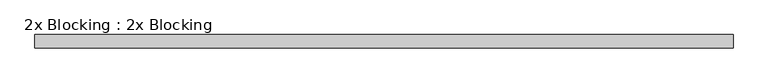
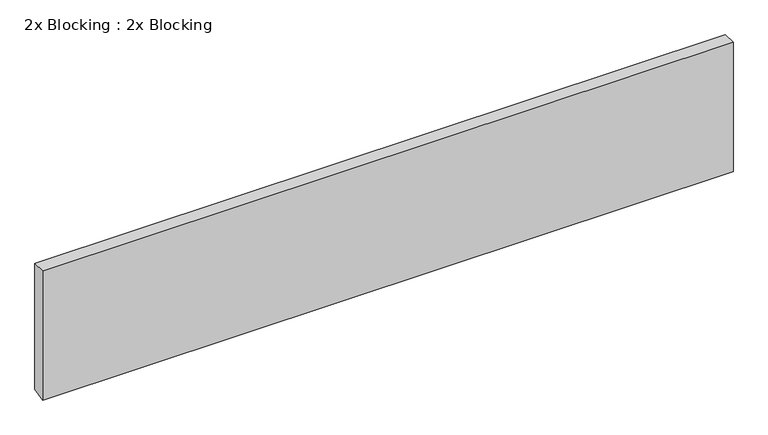
"""IFC4 building model written with IfcOpenShell, lengths in millimetres: proxy geometry, 2x Blocking : 2x Blocking."""

import ifcopenshell
import ifcopenshell.guid

model = None  # the IFC model being written
_history = None  # IfcOwnerHistory: only IFC2X3 demands one
_inside = {}  # id of a spatial element -> (the spatial element, [elements in it])
_under = {}  # id of a project, library or spatial element -> (it, [spatial elements below it])
_declared = {}  # id of a project -> (the project, [libraries it declares])
_typed = {}  # id of a type object -> (the type object, [elements of that type])
_made_of = {}  # id of a material, layer set ... -> (it, [elements and type objects made of it])


def new_model(schema):
    """Start an empty IFC model of exactly this schema.

    Asked for "IFC4X3", IfcOpenShell would pick the latest addendum, in which some entities
    have other attributes; the version numbers below select the first issue.
    IFC2X3 requires an IfcOwnerHistory on every rooted entity: one is made here for all.
    """
    global model, _history
    if schema == "IFC4X3":
        model = ifcopenshell.file(schema_version=(4, 3, 0, 0))
    else:
        model = ifcopenshell.file(schema=schema)
    _inside.clear()
    _under.clear()
    _declared.clear()
    _typed.clear()
    _made_of.clear()
    _history = None
    if model.schema == "IFC2X3":
        org = make("IfcOrganization", Name="unknown")
        user = make(
            "IfcPersonAndOrganization",
            ThePerson=make("IfcPerson", FamilyName="unknown"),
            TheOrganization=org,
        )
        app = make(
            "IfcApplication",
            ApplicationDeveloper=org,
            Version="unknown",
            ApplicationFullName="unknown",
            ApplicationIdentifier="unknown",
        )
        _history = make(
            "IfcOwnerHistory",
            OwningUser=user,
            OwningApplication=app,
            ChangeAction="ADDED",
            CreationDate=0,
        )
    return model


def make(cls, **values):
    """One entity of the class cls with the attributes given. An attribute that is None is left unset."""
    return model.create_entity(
        cls, **{name: value for name, value in values.items() if value is not None}
    )


def rooted(cls, **values):
    """An entity with a GlobalId (a new one), such as an element, a storey or a relation."""
    return make(cls, GlobalId=ifcopenshell.guid.new(), OwnerHistory=_history, **values)


def si_unit(unit_type, name, prefix=None):
    """IfcSIUnit, for example si_unit("LENGTHUNIT", "METRE", prefix="MILLI")."""
    return make("IfcSIUnit", UnitType=unit_type, Prefix=prefix, Name=name)


def assignment(units):
    """IfcUnitAssignment: the units of a project."""
    return None if units is None else make("IfcUnitAssignment", Units=units)


def point(xyz):
    """IfcCartesianPoint."""
    return None if xyz is None else make("IfcCartesianPoint", Coordinates=xyz)


def direction(xyz):
    """IfcDirection."""
    return None if xyz is None else make("IfcDirection", DirectionRatios=xyz)


def frame(location, z_axis=None, x_axis=None):
    """IfcAxis2Placement3D, a coordinate frame: its origin and axes. An axis left out is left unset."""
    return make(
        "IfcAxis2Placement3D",
        Location=point(location),
        Axis=direction(z_axis),
        RefDirection=direction(x_axis),
    )


def origin():
    """The frame at (0, 0, 0) with its axes left unset."""
    return frame((0.0, 0.0, 0.0))


def place(relative_to, where):
    """IfcLocalPlacement: puts the frame where relative to a parent placement (None: the world)."""
    return make(
        "IfcLocalPlacement", PlacementRelTo=relative_to, RelativePlacement=where
    )


def context(
    kind, dimensions, precision=None, world=None, true_north=None, identifier=None
):
    """IfcGeometricRepresentationContext, for example the 3D "Model" context."""
    return make(
        "IfcGeometricRepresentationContext",
        ContextIdentifier=identifier,
        ContextType=kind,
        CoordinateSpaceDimension=dimensions,
        Precision=precision,
        WorldCoordinateSystem=world,
        TrueNorth=true_north,
    )


def project(units=None, contexts=None):
    """IfcProject with its units and contexts."""
    return rooted(
        "IfcProject",
        Name="project",
        RepresentationContexts=contexts,
        UnitsInContext=assignment(units),
    )


def spatial(cls, under=None, at=None, **own):
    """A site, building, storey or space (cls), placed at a placement, below another one or the project."""
    s = rooted(cls, ObjectPlacement=at, **own)
    if under is not None:
        _under.setdefault(under.id(), (under, []))[1].append(s)
    return s


def polyline(points):
    """IfcPolyline through the points."""
    return make("IfcPolyline", Points=[point(p) for p in points])


def outline(outer, holes=None, kind="AREA"):
    """IfcArbitraryClosedProfileDef: a profile drawn as a closed curve; with holes, ...WithVoids."""
    if holes is None:
        return make("IfcArbitraryClosedProfileDef", ProfileType=kind, OuterCurve=outer)
    return make(
        "IfcArbitraryProfileDefWithVoids",
        ProfileType=kind,
        OuterCurve=outer,
        InnerCurves=holes,
    )


def extrude(swept, where, along, depth):
    """IfcExtrudedAreaSolid: the profile swept, set in the frame where, extruded along a direction by depth."""
    return make(
        "IfcExtrudedAreaSolid",
        SweptArea=swept,
        Position=where,
        ExtrudedDirection=direction(along),
        Depth=depth,
    )


def shape(context_of_items, identifier, shape_type, items):
    """IfcShapeRepresentation: the items that make up one representation, for example the "Body"."""
    return make(
        "IfcShapeRepresentation",
        ContextOfItems=context_of_items,
        RepresentationIdentifier=identifier,
        RepresentationType=shape_type,
        Items=items,
    )


def source(mapping_origin, context_of_items, identifier, shape_type, items):
    """IfcRepresentationMap: a shape defined once, which mapped items show again and again."""
    return make(
        "IfcRepresentationMap",
        MappingOrigin=mapping_origin,
        MappedRepresentation=shape(context_of_items, identifier, shape_type, items),
    )


def transform(
    local_origin,
    x_axis=None,
    y_axis=None,
    z_axis=None,
    scale=None,
    scale2=None,
    scale3=None,
    uniform=True,
):
    """IfcCartesianTransformationOperator3D, or its non-uniform kind. x_axis, y_axis, z_axis: its Axis1, 2, 3."""
    if uniform:
        return make(
            "IfcCartesianTransformationOperator3D",
            Axis1=direction(x_axis),
            Axis2=direction(y_axis),
            LocalOrigin=point(local_origin),
            Scale=scale,
            Axis3=direction(z_axis),
        )
    return make(
        "IfcCartesianTransformationOperator3DnonUniform",
        Axis1=direction(x_axis),
        Axis2=direction(y_axis),
        LocalOrigin=point(local_origin),
        Scale=scale,
        Axis3=direction(z_axis),
        Scale2=scale2,
        Scale3=scale3,
    )


def mapped(mapping_source, mapping_target):
    """IfcMappedItem: shows the shape of a source again, moved by a transform."""
    return make(
        "IfcMappedItem", MappingSource=mapping_source, MappingTarget=mapping_target
    )


def made_of(thing, what):
    """Note that an element or type object is made of a material, layer set ...; save() writes the relation."""
    if what is not None:
        _made_of.setdefault(what.id(), (what, []))[1].append(thing)
    return thing


def element(
    cls,
    number,
    at=None,
    inside=None,
    cuts=None,
    type_object=None,
    material=None,
    context=None,
    identifier="Body",
    shape_type=None,
    held_by="IfcProductDefinitionShape",
    body=None,
    shapes=None,
    **own,
):
    """One element of the class cls, such as IfcWall. Its Tag is "e" and its number.

    at: its placement. inside: the storey or other place that contains it. cuts: it is an
    opening in that element (IfcRelVoidsElement). A single representation is given by context,
    identifier, shape_type and body (its items); several are given by shapes. held_by: the class
    of the entity that holds the representations. save() writes the other relations.
    """
    e = rooted(cls, Tag="e%d" % number, ObjectPlacement=at, **own)
    if body is not None:
        shapes = [shape(context, identifier, shape_type, body)]
    if shapes is not None:
        e.Representation = make(held_by, Representations=shapes)
    if inside is not None:
        _inside.setdefault(inside.id(), (inside, []))[1].append(e)
    if cuts is not None:
        rooted(
            "IfcRelVoidsElement", RelatingBuildingElement=cuts, RelatedOpeningElement=e
        )
    if type_object is not None:
        _typed.setdefault(type_object.id(), (type_object, []))[1].append(e)
    return made_of(e, material)


def aggregate(whole, parts):
    """IfcRelAggregates: a whole, such as a stair, and the parts it consists of."""
    return rooted("IfcRelAggregates", RelatingObject=whole, RelatedObjects=parts)


def save(model, path):
    """Write the relations noted so far, then the file.

    IfcRelAggregates (storeys below a building ...), IfcRelContainedInSpatialStructure (elements
    in a storey), IfcRelDefinesByType, IfcRelAssociatesMaterial and IfcRelDeclares: one each for
    every whole, place, type object, material and project.
    """
    for whole, parts in _under.values():
        aggregate(whole, parts)
    for where, things in _inside.values():
        rooted(
            "IfcRelContainedInSpatialStructure",
            RelatedElements=things,
            RelatingStructure=where,
        )
    for kind, things in _typed.values():
        rooted("IfcRelDefinesByType", RelatedObjects=things, RelatingType=kind)
    for what, things in _made_of.values():
        rooted("IfcRelAssociatesMaterial", RelatedObjects=things, RelatingMaterial=what)
    for by, libraries in _declared.values():
        rooted("IfcRelDeclares", RelatingContext=by, RelatedDefinitions=libraries)
    model.write(path)


def proxy_2x_blocking_2x_blocking_7a8122e4(model_context):
    return source(origin(), model_context, "Body", "SweptSolid", [
        extrude(outline(polyline([(-5586.8675368, 42739.1328126), (-5548.7675368, 42739.1328126), (-5548.7675368, 42352.8601703), (-5586.8675368, 42342.8919143), (-5586.8675368, 42739.1328126)])), frame((12382.7678845, 0.0, 0.0), z_axis=(1.0, 0.0, 0.0), x_axis=(0.0, 1.0, 0.0)), (0.0, 0.0, 1.0), 2000.25),
    ])


if __name__ == "__main__":
    model = new_model("IFC4")
    model_context = context("Model", 3, world=origin())
    ifc_project = project(units=[si_unit("LENGTHUNIT", "METRE", prefix="MILLI")], contexts=[model_context])
    site = spatial("IfcSite", under=ifc_project)
    building = spatial("IfcBuilding", under=site)
    placement = place(None, origin())
    proxy_2x_blocking_2x_blocking_shape = proxy_2x_blocking_2x_blocking_7a8122e4(model_context)
    element("IfcBuildingElementProxy", 1, Name="2x Blocking : 2x Blocking", ObjectType="2x Blocking : 2x Blocking", at=placement, inside=building, context=model_context, shape_type="MappedRepresentation", body=[
        mapped(proxy_2x_blocking_2x_blocking_shape, transform((0.0, 0.0, 0.0), x_axis=(1.0, 0.0, 0.0), y_axis=(0.0, 1.0, 0.0), z_axis=(0.0, 0.0, 1.0))),
    ])
    save(model, "model.ifc")

# Revit data of these elements
# Type "2x Blocking : 2x Blocking"
#   NameOverride = "2x Blocking"
# Element 1 (IfcBuildingElementProxy, "2x Blocking : 2x Blocking")
#   Materials on its faces: "2X BLOCKING AS REQUIRED"
# Materials
#   "2X BLOCKING AS REQUIRED": class "Unassigned", colour RGB 166 124 85, transparency 0, Cost = 0
